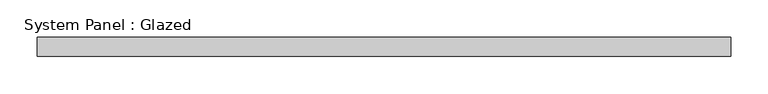
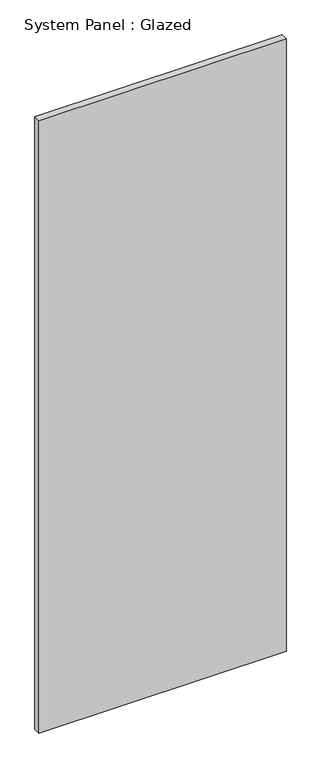
"""IFC4 building model written with IfcOpenShell, lengths in millimetres: plate geometry, System Panel : Glazed."""

import ifcopenshell
import ifcopenshell.guid

model = None  # the IFC model being written
_history = None  # IfcOwnerHistory: only IFC2X3 demands one
_inside = {}  # id of a spatial element -> (the spatial element, [elements in it])
_under = {}  # id of a project, library or spatial element -> (it, [spatial elements below it])
_declared = {}  # id of a project -> (the project, [libraries it declares])
_typed = {}  # id of a type object -> (the type object, [elements of that type])
_made_of = {}  # id of a material, layer set ... -> (it, [elements and type objects made of it])


def new_model(schema):
    """Start an empty IFC model of exactly this schema.

    Asked for "IFC4X3", IfcOpenShell would pick the latest addendum, in which some entities
    have other attributes; the version numbers below select the first issue.
    IFC2X3 requires an IfcOwnerHistory on every rooted entity: one is made here for all.
    """
    global model, _history
    if schema == "IFC4X3":
        model = ifcopenshell.file(schema_version=(4, 3, 0, 0))
    else:
        model = ifcopenshell.file(schema=schema)
    _inside.clear()
    _under.clear()
    _declared.clear()
    _typed.clear()
    _made_of.clear()
    _history = None
    if model.schema == "IFC2X3":
        org = make("IfcOrganization", Name="unknown")
        user = make(
            "IfcPersonAndOrganization",
            ThePerson=make("IfcPerson", FamilyName="unknown"),
            TheOrganization=org,
        )
        app = make(
            "IfcApplication",
            ApplicationDeveloper=org,
            Version="unknown",
            ApplicationFullName="unknown",
            ApplicationIdentifier="unknown",
        )
        _history = make(
            "IfcOwnerHistory",
            OwningUser=user,
            OwningApplication=app,
            ChangeAction="ADDED",
            CreationDate=0,
        )
    return model


def make(cls, **values):
    """One entity of the class cls with the attributes given. An attribute that is None is left unset."""
    return model.create_entity(
        cls, **{name: value for name, value in values.items() if value is not None}
    )


def rooted(cls, **values):
    """An entity with a GlobalId (a new one), such as an element, a storey or a relation."""
    return make(cls, GlobalId=ifcopenshell.guid.new(), OwnerHistory=_history, **values)


def si_unit(unit_type, name, prefix=None):
    """IfcSIUnit, for example si_unit("LENGTHUNIT", "METRE", prefix="MILLI")."""
    return make("IfcSIUnit", UnitType=unit_type, Prefix=prefix, Name=name)


def assignment(units):
    """IfcUnitAssignment: the units of a project."""
    return None if units is None else make("IfcUnitAssignment", Units=units)


def point(xyz):
    """IfcCartesianPoint."""
    return None if xyz is None else make("IfcCartesianPoint", Coordinates=xyz)


def direction(xyz):
    """IfcDirection."""
    return None if xyz is None else make("IfcDirection", DirectionRatios=xyz)


def frame(location, z_axis=None, x_axis=None):
    """IfcAxis2Placement3D, a coordinate frame: its origin and axes. An axis left out is left unset."""
    return make(
        "IfcAxis2Placement3D",
        Location=point(location),
        Axis=direction(z_axis),
        RefDirection=direction(x_axis),
    )


def origin():
    """The frame at (0, 0, 0) with its axes left unset."""
    return frame((0.0, 0.0, 0.0))


def origin_with_axes():
    """The frame at (0, 0, 0) with the z axis (0, 0, 1) and the x axis (1, 0, 0) written out."""
    return frame((0.0, 0.0, 0.0), z_axis=(0.0, 0.0, 1.0), x_axis=(1.0, 0.0, 0.0))


def place(relative_to, where):
    """IfcLocalPlacement: puts the frame where relative to a parent placement (None: the world)."""
    return make(
        "IfcLocalPlacement", PlacementRelTo=relative_to, RelativePlacement=where
    )


def context(
    kind, dimensions, precision=None, world=None, true_north=None, identifier=None
):
    """IfcGeometricRepresentationContext, for example the 3D "Model" context."""
    return make(
        "IfcGeometricRepresentationContext",
        ContextIdentifier=identifier,
        ContextType=kind,
        CoordinateSpaceDimension=dimensions,
        Precision=precision,
        WorldCoordinateSystem=world,
        TrueNorth=true_north,
    )


def project(units=None, contexts=None):
    """IfcProject with its units and contexts."""
    return rooted(
        "IfcProject",
        Name="project",
        RepresentationContexts=contexts,
        UnitsInContext=assignment(units),
    )


def spatial(cls, under=None, at=None, **own):
    """A site, building, storey or space (cls), placed at a placement, below another one or the project."""
    s = rooted(cls, ObjectPlacement=at, **own)
    if under is not None:
        _under.setdefault(under.id(), (under, []))[1].append(s)
    return s


def polyline(points):
    """IfcPolyline through the points."""
    return make("IfcPolyline", Points=[point(p) for p in points])


def outline(outer, holes=None, kind="AREA"):
    """IfcArbitraryClosedProfileDef: a profile drawn as a closed curve; with holes, ...WithVoids."""
    if holes is None:
        return make("IfcArbitraryClosedProfileDef", ProfileType=kind, OuterCurve=outer)
    return make(
        "IfcArbitraryProfileDefWithVoids",
        ProfileType=kind,
        OuterCurve=outer,
        InnerCurves=holes,
    )


def extrude(swept, where, along, depth):
    """IfcExtrudedAreaSolid: the profile swept, set in the frame where, extruded along a direction by depth."""
    return make(
        "IfcExtrudedAreaSolid",
        SweptArea=swept,
        Position=where,
        ExtrudedDirection=direction(along),
        Depth=depth,
    )


def shape(context_of_items, identifier, shape_type, items):
    """IfcShapeRepresentation: the items that make up one representation, for example the "Body"."""
    return make(
        "IfcShapeRepresentation",
        ContextOfItems=context_of_items,
        RepresentationIdentifier=identifier,
        RepresentationType=shape_type,
        Items=items,
    )


def source(mapping_origin, context_of_items, identifier, shape_type, items):
    """IfcRepresentationMap: a shape defined once, which mapped items show again and again."""
    return make(
        "IfcRepresentationMap",
        MappingOrigin=mapping_origin,
        MappedRepresentation=shape(context_of_items, identifier, shape_type, items),
    )


def transform(
    local_origin,
    x_axis=None,
    y_axis=None,
    z_axis=None,
    scale=None,
    scale2=None,
    scale3=None,
    uniform=True,
):
    """IfcCartesianTransformationOperator3D, or its non-uniform kind. x_axis, y_axis, z_axis: its Axis1, 2, 3."""
    if uniform:
        return make(
            "IfcCartesianTransformationOperator3D",
            Axis1=direction(x_axis),
            Axis2=direction(y_axis),
            LocalOrigin=point(local_origin),
            Scale=scale,
            Axis3=direction(z_axis),
        )
    return make(
        "IfcCartesianTransformationOperator3DnonUniform",
        Axis1=direction(x_axis),
        Axis2=direction(y_axis),
        LocalOrigin=point(local_origin),
        Scale=scale,
        Axis3=direction(z_axis),
        Scale2=scale2,
        Scale3=scale3,
    )


def mapped(mapping_source, mapping_target):
    """IfcMappedItem: shows the shape of a source again, moved by a transform."""
    return make(
        "IfcMappedItem", MappingSource=mapping_source, MappingTarget=mapping_target
    )


def made_of(thing, what):
    """Note that an element or type object is made of a material, layer set ...; save() writes the relation."""
    if what is not None:
        _made_of.setdefault(what.id(), (what, []))[1].append(thing)
    return thing


def element(
    cls,
    number,
    at=None,
    inside=None,
    cuts=None,
    type_object=None,
    material=None,
    context=None,
    identifier="Body",
    shape_type=None,
    held_by="IfcProductDefinitionShape",
    body=None,
    shapes=None,
    **own,
):
    """One element of the class cls, such as IfcWall. Its Tag is "e" and its number.

    at: its placement. inside: the storey or other place that contains it. cuts: it is an
    opening in that element (IfcRelVoidsElement). A single representation is given by context,
    identifier, shape_type and body (its items); several are given by shapes. held_by: the class
    of the entity that holds the representations. save() writes the other relations.
    """
    e = rooted(cls, Tag="e%d" % number, ObjectPlacement=at, **own)
    if body is not None:
        shapes = [shape(context, identifier, shape_type, body)]
    if shapes is not None:
        e.Representation = make(held_by, Representations=shapes)
    if inside is not None:
        _inside.setdefault(inside.id(), (inside, []))[1].append(e)
    if cuts is not None:
        rooted(
            "IfcRelVoidsElement", RelatingBuildingElement=cuts, RelatedOpeningElement=e
        )
    if type_object is not None:
        _typed.setdefault(type_object.id(), (type_object, []))[1].append(e)
    return made_of(e, material)


def aggregate(whole, parts):
    """IfcRelAggregates: a whole, such as a stair, and the parts it consists of."""
    return rooted("IfcRelAggregates", RelatingObject=whole, RelatedObjects=parts)


def save(model, path):
    """Write the relations noted so far, then the file.

    IfcRelAggregates (storeys below a building ...), IfcRelContainedInSpatialStructure (elements
    in a storey), IfcRelDefinesByType, IfcRelAssociatesMaterial and IfcRelDeclares: one each for
    every whole, place, type object, material and project.
    """
    for whole, parts in _under.values():
        aggregate(whole, parts)
    for where, things in _inside.values():
        rooted(
            "IfcRelContainedInSpatialStructure",
            RelatedElements=things,
            RelatingStructure=where,
        )
    for kind, things in _typed.values():
        rooted("IfcRelDefinesByType", RelatedObjects=things, RelatingType=kind)
    for what, things in _made_of.values():
        rooted("IfcRelAssociatesMaterial", RelatedObjects=things, RelatingMaterial=what)
    for by, libraries in _declared.values():
        rooted("IfcRelDeclares", RelatingContext=by, RelatedDefinitions=libraries)
    model.write(path)


def system_panel_glazed_7cecf9c6(model_context):
    return source(origin(), model_context, "Body", "SweptSolid", [
        extrude(outline(polyline([(462.5, 24.5), (-462.5, 24.5), (-462.5, 49.5), (462.5, 49.5), (462.5, 24.5)])), origin_with_axes(), (0.0, 0.0, 1.0), 2422.0381538),
    ])


if __name__ == "__main__":
    model = new_model("IFC4")
    model_context = context("Model", 3, world=origin())
    ifc_project = project(units=[si_unit("LENGTHUNIT", "METRE", prefix="MILLI")], contexts=[model_context])
    site = spatial("IfcSite", under=ifc_project)
    building = spatial("IfcBuilding", under=site)
    placement = place(None, origin())
    system_panel_glazed_shape = system_panel_glazed_7cecf9c6(model_context)
    element("IfcPlate", 1, ObjectType="System Panel : Glazed", at=placement, inside=building, context=model_context, shape_type="MappedRepresentation", body=[
        mapped(system_panel_glazed_shape, transform((0.0, 0.0, 0.0), x_axis=(1.0, 0.0, 0.0), y_axis=(0.0, 1.0, 0.0), z_axis=(0.0, 0.0, 1.0))),
    ])
    save(model, "model.ifc")

# Revit data of these elements
# Type "System Panel : Glazed"
#   Keynote = "H11"
#   Construction Type Id = "GSP4R"
#   Analytic Construction = "1/8 in Pilkington single glazing"
#   Visual Light Transmittance = 0.9
#   Solar Heat Gain Coefficient = 0.86
#   Heat Transfer Coefficient (U) = 6.7069 W/(m²·K)
#   Define Thermal Properties by = 1
# Element 1 (IfcPlate, "System Panel : Glazed")
#   Materials on its faces: "Glass"
# Materials
#   "Glass": class "Glass", colour RGB 0 128 192, transparency 0.9, Description = "Soda Lime Glass", Cost = 0
